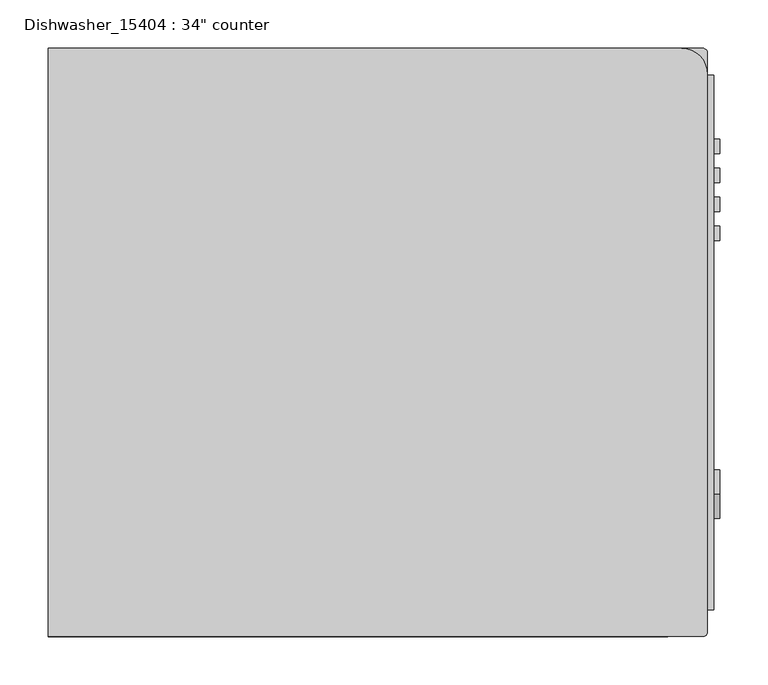
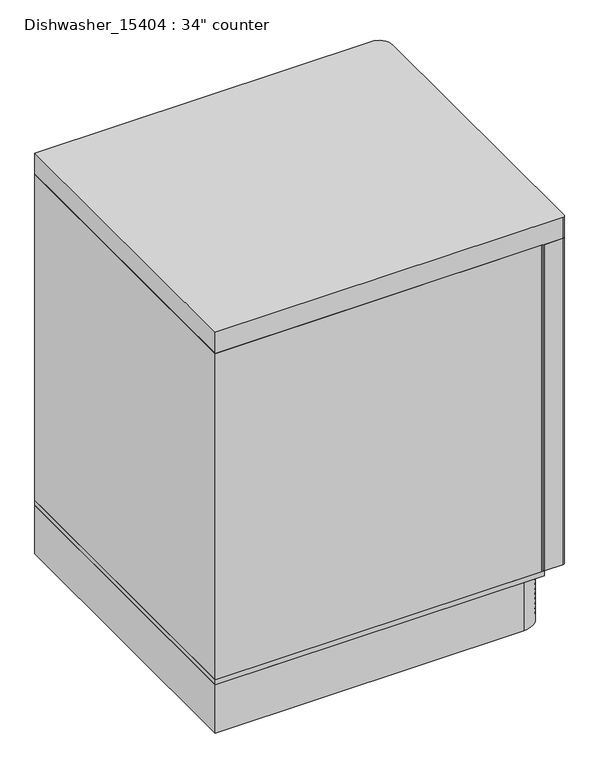
"""IFC4 building model written with IfcOpenShell, lengths in millimetres: proxy geometry."""

import ifcopenshell
import ifcopenshell.guid

model = None  # the IFC model being written
_history = None  # IfcOwnerHistory: only IFC2X3 demands one
_inside = {}  # id of a spatial element -> (the spatial element, [elements in it])
_under = {}  # id of a project, library or spatial element -> (it, [spatial elements below it])
_declared = {}  # id of a project -> (the project, [libraries it declares])
_typed = {}  # id of a type object -> (the type object, [elements of that type])
_made_of = {}  # id of a material, layer set ... -> (it, [elements and type objects made of it])


def new_model(schema):
    """Start an empty IFC model of exactly this schema.

    Asked for "IFC4X3", IfcOpenShell would pick the latest addendum, in which some entities
    have other attributes; the version numbers below select the first issue.
    IFC2X3 requires an IfcOwnerHistory on every rooted entity: one is made here for all.
    """
    global model, _history
    if schema == "IFC4X3":
        model = ifcopenshell.file(schema_version=(4, 3, 0, 0))
    else:
        model = ifcopenshell.file(schema=schema)
    _inside.clear()
    _under.clear()
    _declared.clear()
    _typed.clear()
    _made_of.clear()
    _history = None
    if model.schema == "IFC2X3":
        org = make("IfcOrganization", Name="unknown")
        user = make(
            "IfcPersonAndOrganization",
            ThePerson=make("IfcPerson", FamilyName="unknown"),
            TheOrganization=org,
        )
        app = make(
            "IfcApplication",
            ApplicationDeveloper=org,
            Version="unknown",
            ApplicationFullName="unknown",
            ApplicationIdentifier="unknown",
        )
        _history = make(
            "IfcOwnerHistory",
            OwningUser=user,
            OwningApplication=app,
            ChangeAction="ADDED",
            CreationDate=0,
        )
    return model


def make(cls, **values):
    """One entity of the class cls with the attributes given. An attribute that is None is left unset."""
    return model.create_entity(
        cls, **{name: value for name, value in values.items() if value is not None}
    )


def rooted(cls, **values):
    """An entity with a GlobalId (a new one), such as an element, a storey or a relation."""
    return make(cls, GlobalId=ifcopenshell.guid.new(), OwnerHistory=_history, **values)


def si_unit(unit_type, name, prefix=None):
    """IfcSIUnit, for example si_unit("LENGTHUNIT", "METRE", prefix="MILLI")."""
    return make("IfcSIUnit", UnitType=unit_type, Prefix=prefix, Name=name)


def assignment(units):
    """IfcUnitAssignment: the units of a project."""
    return None if units is None else make("IfcUnitAssignment", Units=units)


def point(xyz):
    """IfcCartesianPoint."""
    return None if xyz is None else make("IfcCartesianPoint", Coordinates=xyz)


def direction(xyz):
    """IfcDirection."""
    return None if xyz is None else make("IfcDirection", DirectionRatios=xyz)


def frame(location, z_axis=None, x_axis=None):
    """IfcAxis2Placement3D, a coordinate frame: its origin and axes. An axis left out is left unset."""
    return make(
        "IfcAxis2Placement3D",
        Location=point(location),
        Axis=direction(z_axis),
        RefDirection=direction(x_axis),
    )


def frame_2d(location, x_axis=None):
    """IfcAxis2Placement2D, a coordinate frame in the plane: its origin and x axis."""
    return make(
        "IfcAxis2Placement2D", Location=point(location), RefDirection=direction(x_axis)
    )


def origin():
    """The frame at (0, 0, 0) with its axes left unset."""
    return frame((0.0, 0.0, 0.0))


def place(relative_to, where):
    """IfcLocalPlacement: puts the frame where relative to a parent placement (None: the world)."""
    return make(
        "IfcLocalPlacement", PlacementRelTo=relative_to, RelativePlacement=where
    )


def context(
    kind, dimensions, precision=None, world=None, true_north=None, identifier=None
):
    """IfcGeometricRepresentationContext, for example the 3D "Model" context."""
    return make(
        "IfcGeometricRepresentationContext",
        ContextIdentifier=identifier,
        ContextType=kind,
        CoordinateSpaceDimension=dimensions,
        Precision=precision,
        WorldCoordinateSystem=world,
        TrueNorth=true_north,
    )


def project(units=None, contexts=None):
    """IfcProject with its units and contexts."""
    return rooted(
        "IfcProject",
        Name="project",
        RepresentationContexts=contexts,
        UnitsInContext=assignment(units),
    )


def spatial(cls, under=None, at=None, **own):
    """A site, building, storey or space (cls), placed at a placement, below another one or the project."""
    s = rooted(cls, ObjectPlacement=at, **own)
    if under is not None:
        _under.setdefault(under.id(), (under, []))[1].append(s)
    return s


def polyline(points):
    """IfcPolyline through the points."""
    return make("IfcPolyline", Points=[point(p) for p in points])


def circle_curve(where, radius):
    """IfcCircle in the frame where."""
    return make("IfcCircle", Position=where, Radius=radius)


def trimmed(basis, trim1, trim2, sense, master):
    """IfcTrimmedCurve: the piece of a basis curve between two trims."""
    return make(
        "IfcTrimmedCurve",
        BasisCurve=basis,
        Trim1=trim1,
        Trim2=trim2,
        SenseAgreement=sense,
        MasterRepresentation=master,
    )


def segment(curve, same_sense, transition):
    """IfcCompositeCurveSegment."""
    return make(
        "IfcCompositeCurveSegment",
        Transition=transition,
        SameSense=same_sense,
        ParentCurve=curve,
    )


def composite_curve(segments, self_intersect=None):
    """IfcCompositeCurve: segments joined end to end."""
    return make("IfcCompositeCurve", Segments=segments, SelfIntersect=self_intersect)


def outline(outer, holes=None, kind="AREA"):
    """IfcArbitraryClosedProfileDef: a profile drawn as a closed curve; with holes, ...WithVoids."""
    if holes is None:
        return make("IfcArbitraryClosedProfileDef", ProfileType=kind, OuterCurve=outer)
    return make(
        "IfcArbitraryProfileDefWithVoids",
        ProfileType=kind,
        OuterCurve=outer,
        InnerCurves=holes,
    )


def extrude(swept, where, along, depth):
    """IfcExtrudedAreaSolid: the profile swept, set in the frame where, extruded along a direction by depth."""
    return make(
        "IfcExtrudedAreaSolid",
        SweptArea=swept,
        Position=where,
        ExtrudedDirection=direction(along),
        Depth=depth,
    )


def shape(context_of_items, identifier, shape_type, items):
    """IfcShapeRepresentation: the items that make up one representation, for example the "Body"."""
    return make(
        "IfcShapeRepresentation",
        ContextOfItems=context_of_items,
        RepresentationIdentifier=identifier,
        RepresentationType=shape_type,
        Items=items,
    )


def source(mapping_origin, context_of_items, identifier, shape_type, items):
    """IfcRepresentationMap: a shape defined once, which mapped items show again and again."""
    return make(
        "IfcRepresentationMap",
        MappingOrigin=mapping_origin,
        MappedRepresentation=shape(context_of_items, identifier, shape_type, items),
    )


def transform(
    local_origin,
    x_axis=None,
    y_axis=None,
    z_axis=None,
    scale=None,
    scale2=None,
    scale3=None,
    uniform=True,
):
    """IfcCartesianTransformationOperator3D, or its non-uniform kind. x_axis, y_axis, z_axis: its Axis1, 2, 3."""
    if uniform:
        return make(
            "IfcCartesianTransformationOperator3D",
            Axis1=direction(x_axis),
            Axis2=direction(y_axis),
            LocalOrigin=point(local_origin),
            Scale=scale,
            Axis3=direction(z_axis),
        )
    return make(
        "IfcCartesianTransformationOperator3DnonUniform",
        Axis1=direction(x_axis),
        Axis2=direction(y_axis),
        LocalOrigin=point(local_origin),
        Scale=scale,
        Axis3=direction(z_axis),
        Scale2=scale2,
        Scale3=scale3,
    )


def mapped(mapping_source, mapping_target):
    """IfcMappedItem: shows the shape of a source again, moved by a transform."""
    return make(
        "IfcMappedItem", MappingSource=mapping_source, MappingTarget=mapping_target
    )


def made_of(thing, what):
    """Note that an element or type object is made of a material, layer set ...; save() writes the relation."""
    if what is not None:
        _made_of.setdefault(what.id(), (what, []))[1].append(thing)
    return thing


def element(
    cls,
    number,
    at=None,
    inside=None,
    cuts=None,
    type_object=None,
    material=None,
    context=None,
    identifier="Body",
    shape_type=None,
    held_by="IfcProductDefinitionShape",
    body=None,
    shapes=None,
    **own,
):
    """One element of the class cls, such as IfcWall. Its Tag is "e" and its number.

    at: its placement. inside: the storey or other place that contains it. cuts: it is an
    opening in that element (IfcRelVoidsElement). A single representation is given by context,
    identifier, shape_type and body (its items); several are given by shapes. held_by: the class
    of the entity that holds the representations. save() writes the other relations.
    """
    e = rooted(cls, Tag="e%d" % number, ObjectPlacement=at, **own)
    if body is not None:
        shapes = [shape(context, identifier, shape_type, body)]
    if shapes is not None:
        e.Representation = make(held_by, Representations=shapes)
    if inside is not None:
        _inside.setdefault(inside.id(), (inside, []))[1].append(e)
    if cuts is not None:
        rooted(
            "IfcRelVoidsElement", RelatingBuildingElement=cuts, RelatedOpeningElement=e
        )
    if type_object is not None:
        _typed.setdefault(type_object.id(), (type_object, []))[1].append(e)
    return made_of(e, material)


def aggregate(whole, parts):
    """IfcRelAggregates: a whole, such as a stair, and the parts it consists of."""
    return rooted("IfcRelAggregates", RelatingObject=whole, RelatedObjects=parts)


def save(model, path):
    """Write the relations noted so far, then the file.

    IfcRelAggregates (storeys below a building ...), IfcRelContainedInSpatialStructure (elements
    in a storey), IfcRelDefinesByType, IfcRelAssociatesMaterial and IfcRelDeclares: one each for
    every whole, place, type object, material and project.
    """
    for whole, parts in _under.values():
        aggregate(whole, parts)
    for where, things in _inside.values():
        rooted(
            "IfcRelContainedInSpatialStructure",
            RelatedElements=things,
            RelatingStructure=where,
        )
    for kind, things in _typed.values():
        rooted("IfcRelDefinesByType", RelatedObjects=things, RelatingType=kind)
    for what, things in _made_of.values():
        rooted("IfcRelAssociatesMaterial", RelatedObjects=things, RelatingMaterial=what)
    for by, libraries in _declared.values():
        rooted("IfcRelDeclares", RelatingContext=by, RelatedDefinitions=libraries)
    model.write(path)


def plane_surface(at):
    """IfcPlane: the flat surface through the origin of the frame at, square to its z axis."""
    return make("IfcPlane", Position=at)


def cylinder_surface(at, radius):
    """IfcCylindricalSurface: all points at the distance radius from the z axis of the frame at."""
    return make("IfcCylindricalSurface", Position=at, Radius=radius)


def advanced_brep(points, edges, surfaces, faces):
    """IfcAdvancedBrep: a solid bounded by faces that lie on surfaces and meet in shared edges.

    An edge is (start, end): straight between two places in points (the first is 0);
    or (start, end, curve); or (start, end, curve, False) where it runs against its curve.
    A face is (place in surfaces, loops), or (place, loops, False) where it looks against
    its surface's normal. A loop lists edges by number (the first is 1), with a minus sign
    where the edge is run from its end to its start. The first loop is the outer one.
    """
    corners = [point(p) for p in points]
    vertices = [make("IfcVertexPoint", VertexGeometry=c) for c in corners]
    made = []
    for start, end, *more in edges:
        made.append(
            make(
                "IfcEdgeCurve",
                EdgeStart=vertices[start],
                EdgeEnd=vertices[end],
                EdgeGeometry=more[0] if more else make("IfcPolyline", Points=[corners[start], corners[end]]),
                SameSense=more[1] if len(more) > 1 else True,
            )
        )
    hull = []
    for where, loops, *sense in faces:
        bounds = []
        for j, loop in enumerate(loops):
            ring = [make("IfcOrientedEdge", EdgeElement=made[abs(k) - 1], Orientation=k > 0) for k in loop]
            bounds.append(
                make(
                    "IfcFaceOuterBound" if j == 0 else "IfcFaceBound",
                    Bound=make("IfcEdgeLoop", EdgeList=ring),
                    Orientation=True,
                )
            )
        hull.append(make("IfcAdvancedFace", Bounds=bounds, FaceSurface=surfaces[where], SameSense=sense[0] if sense else True))
    return make("IfcAdvancedBrep", Outer=make("IfcClosedShell", CfsFaces=hull))


def proxy_e1c3c540(model_context):
    return source(origin(), model_context, "Body", "SolidModel", [
        extrude(outline(composite_curve([segment(trimmed(circle_curve(frame_2d((147.53066, 741.5840355)), 25.0), [point((147.53066, 716.5840355))], [point((147.53066, 766.5840355))], False, "CARTESIAN"), True, "CONTINUOUS"), segment(trimmed(circle_curve(frame_2d((147.53066, 741.5840355)), 25.0), [point((147.53066, 766.5840355))], [point((147.53066, 716.5840355))], False, "CARTESIAN"), True, "CONTINUOUS")], self_intersect=False)), frame((688.975, 0.0, 0.0), z_axis=(1.0, 0.0, 0.0), x_axis=(0.0, 1.0, 0.0)), (0.0, 0.0, 1.0), 6.35),
        extrude(outline(polyline([(688.975, 410.2108979), (688.975, 425.2108979), (695.325, 425.2108979), (695.325, 410.2108979), (688.975, 410.2108979)])), frame((0.0, 0.0, 745.4030607), z_axis=(0.0, 0.0, 1.0), x_axis=(1.0, 0.0, 0.0)), (0.0, 0.0, 1.0), 15.0),
        extrude(outline(polyline([(688.975, 440.2108979), (688.975, 455.2108979), (695.325, 455.2108979), (695.325, 440.2108979), (688.975, 440.2108979)])), frame((0.0, 0.0, 745.4030607), z_axis=(0.0, 0.0, 1.0), x_axis=(1.0, 0.0, 0.0)), (0.0, 0.0, 1.0), 15.0),
        extrude(outline(polyline([(688.975, 470.2108979), (688.975, 485.2108979), (695.325, 485.2108979), (695.325, 470.2108979), (688.975, 470.2108979)])), frame((0.0, 0.0, 745.4030607), z_axis=(0.0, 0.0, 1.0), x_axis=(1.0, 0.0, 0.0)), (0.0, 0.0, 1.0), 15.0),
        extrude(outline(polyline([(688.975, 500.2108979), (688.975, 515.2108979), (695.325, 515.2108979), (695.325, 500.2108979), (688.975, 500.2108979)])), frame((0.0, 0.0, 745.4030607), z_axis=(0.0, 0.0, 1.0), x_axis=(1.0, 0.0, 0.0)), (0.0, 0.0, 1.0), 15.0),
        extrude(outline(composite_curve([segment(polyline([(512.7209143, 694.5980964), (96.8794309, 694.5980964)]), True, "CONTINUOUS"), segment(trimmed(circle_curve(frame_2d((96.8794309, 729.5980964)), 35.0), [point((96.8794309, 694.5980964))], [point((66.2677412, 712.6297597))], False, "CARTESIAN"), True, "CONTINUOUS"), segment(polyline([(66.2677412, 712.6297597), (27.7608134, 782.0980964), (581.8395319, 782.0980964), (543.3326041, 712.6297597)]), True, "CONTINUOUS"), segment(trimmed(circle_curve(frame_2d((512.7209143, 729.5980964)), 35.0), [point((543.3326041, 712.6297597))], [point((512.7209143, 694.5980964))], False, "CARTESIAN"), True, "CONTINUOUS")], self_intersect=False)), frame((638.175, 0.0, 0.0), z_axis=(1.0, 0.0, 0.0), x_axis=(0.0, 1.0, 0.0)), (0.0, 0.0, 1.0), 50.8),
        extrude(outline(composite_curve([segment(polyline([(0.0, 609.6), (636.35, 609.6)]), True, "CONTINUOUS"), segment(trimmed(circle_curve(frame_2d((636.35, 604.6)), 5.0), [point((636.35, 609.6))], [point((641.35, 604.6))], False, "CARTESIAN"), True, "CONTINUOUS"), segment(polyline([(641.35, 604.6), (641.35, 5.0003453)]), True, "CONTINUOUS"), segment(trimmed(circle_curve(frame_2d((636.35, 5.0003453)), 5.0), [point((641.35, 5.0003453))], [point((636.35, 0.0003453))], False, "CARTESIAN"), True, "CONTINUOUS"), segment(polyline([(636.35, 0.0003453), (0.0, 0.0003453), (0.0, 609.6)]), True, "CONTINUOUS")], self_intersect=False)), frame((0.0, 0.0, 110.0), z_axis=(0.0, 0.0, 1.0), x_axis=(1.0, 0.0, 0.0)), (0.0, 0.0, 1.0), 672.0980964),
        extrude(outline(composite_curve([segment(polyline([(0.0, 609.6), (655.4, 609.6)]), True, "CONTINUOUS"), segment(trimmed(circle_curve(frame_2d((655.4, 582.375)), 27.225), [point((655.4, 609.6))], [point((682.625, 582.375))], False, "CARTESIAN"), True, "CONTINUOUS"), segment(polyline([(682.625, 582.375), (682.625, 5.0)]), True, "CONTINUOUS"), segment(trimmed(circle_curve(frame_2d((677.625, 5.0)), 5.0), [point((682.625, 5.0))], [point((677.625, 0.0))], False, "CARTESIAN"), True, "CONTINUOUS"), segment(polyline([(677.625, 0.0), (0.0, 0.0), (0.0, 609.6)]), True, "CONTINUOUS")], self_intersect=False)), frame((0.0, 0.0, 782.0980964), z_axis=(0.0, 0.0, 1.0), x_axis=(1.0, 0.0, 0.0)), (0.0, 0.0, 1.0), 43.4019036),
        extrude(outline(composite_curve([segment(polyline([(641.35, 609.6), (677.625, 609.6)]), True, "CONTINUOUS"), segment(trimmed(circle_curve(frame_2d((677.625, 604.6)), 5.0), [point((677.625, 609.6))], [point((682.625, 604.6))], False, "CARTESIAN"), True, "CONTINUOUS"), segment(polyline([(682.625, 604.6), (682.625, 5.0)]), True, "CONTINUOUS"), segment(trimmed(circle_curve(frame_2d((677.625, 5.0)), 5.0), [point((682.625, 5.0))], [point((677.625, 0.0))], False, "CARTESIAN"), True, "CONTINUOUS"), segment(polyline([(677.625, 0.0), (641.35, 0.0), (641.35, 609.6)]), True, "CONTINUOUS")], self_intersect=False)), frame((0.0, 0.0, 110.0), z_axis=(0.0, 0.0, 1.0), x_axis=(1.0, 0.0, 0.0)), (0.0, 0.0, 1.0), 672.0980964),
        extrude(outline(polyline([(0.0, 609.6), (641.35, 609.6), (641.35, 0.0), (0.0, 0.0), (0.0, 609.6)])), frame((0.0, 0.0, 100.0), z_axis=(0.0, 0.0, 1.0), x_axis=(1.0, 0.0, 0.0)), (0.0, 0.0, 1.0), 10.0),
        advanced_brep(
        [(0.0, 609.6, 100.0), (0.0, 0.0, 100.0), (601.35, 0.0, 100.0), (641.35, 40.0, 100.0), (641.35, 569.6, 100.0), (601.35, 609.6, 100.0), (0.0, 609.6, 0.0), (601.35, 609.6, 0.0), (641.35, 569.6, 0.0), (641.35, 40.0, 0.0), (601.35, 0.0, 0.0), (0.0, 0.0, 0.0), (641.35, 40.0, 16.3757772), (628.65, 10.7645763, 16.3757772), (628.65, 10.7645763, 21.3757772), (641.35, 40.0, 21.3757772), (641.35, 40.0, 26.2238547), (628.65, 10.7645763, 26.2238547), (628.65, 10.7645763, 31.2238547), (641.35, 40.0, 31.2238547), (641.35, 40.0, 36.2238547), (628.65, 10.7645763, 36.2238547), (628.65, 10.7645763, 41.2238547), (641.35, 40.0, 41.2238547), (641.35, 40.0, 46.2238547), (628.65, 10.7645763, 46.2238547), (628.65, 10.7645763, 51.2238547), (641.35, 40.0, 51.2238547), (641.35, 40.0, 56.2238547), (628.65, 10.7645763, 56.2238547), (628.65, 10.7645763, 61.2238547), (641.35, 40.0, 61.2238547), (641.35, 40.0, 66.2238547), (628.65, 10.7645763, 66.2238547), (628.65, 10.7645763, 71.2238547), (641.35, 40.0, 71.2238547), (641.35, 40.0, 76.2238547), (628.65, 10.7645763, 76.2238547), (628.65, 10.7645763, 81.2238547), (641.35, 40.0, 81.2238547), (641.35, 40.0, 86.2238547), (628.65, 10.7645763, 86.2238547), (628.65, 10.7645763, 91.2238547), (641.35, 40.0, 91.2238547), (641.35, 569.6, 91.2238547), (641.35, 569.6, 16.3757772), (641.35, 569.6, 21.3757772), (641.35, 569.6, 26.2238547), (641.35, 569.6, 31.2238547), (641.35, 569.6, 36.2238547), (641.35, 569.6, 41.2238547), (641.35, 569.6, 46.2238547), (641.35, 569.6, 51.2238547), (641.35, 569.6, 56.2238547), (641.35, 569.6, 61.2238547), (641.35, 569.6, 66.2238547), (641.35, 569.6, 71.2238547), (641.35, 569.6, 76.2238547), (641.35, 569.6, 81.2238547), (641.35, 569.6, 86.2238547), (628.65, 598.8354237, 91.2238547), (628.65, 598.8354237, 86.2238547), (628.65, 598.8354237, 81.2238547), (628.65, 598.8354237, 76.2238547), (628.65, 598.8354237, 71.2238547), (628.65, 598.8354237, 66.2238547), (628.65, 598.8354237, 61.2238547), (628.65, 598.8354237, 56.2238547), (628.65, 598.8354237, 51.2238547), (628.65, 598.8354237, 46.2238547), (628.65, 598.8354237, 41.2238547), (628.65, 598.8354237, 36.2238547), (628.65, 598.8354237, 31.2238547), (628.65, 598.8354237, 26.2238547), (628.65, 598.8354237, 21.3757772), (628.65, 598.8354237, 16.3757772)],
        [
            (0, 1),
            (1, 2),
            (2, 3, circle_curve(frame((601.35, 40.0, 100.0), z_axis=(0.0, 0.0, 1.0), x_axis=(1.0, 0.0, 0.0)), 40.0)),
            (3, 4),
            (4, 5, circle_curve(frame((601.35, 569.6, 100.0), z_axis=(0.0, 0.0, 1.0), x_axis=(1.0, 0.0, 0.0)), 40.0)),
            (5, 0),
            (6, 7),
            (7, 8, circle_curve(frame((601.35, 569.6, 0.0), z_axis=(0.0, 0.0, -1.0), x_axis=(1.0, 0.0, 0.0)), 40.0)),
            (8, 9),
            (9, 10, circle_curve(frame((601.35, 40.0, 0.0), z_axis=(0.0, 0.0, -1.0), x_axis=(1.0, 0.0, 0.0)), 40.0)),
            (10, 11),
            (11, 6),
            (0, 6),
            (11, 1),
            (10, 2),
            (9, 12),
            (12, 13, circle_curve(frame((601.35, 40.0, 16.3757772), z_axis=(0.0, 0.0, -1.0), x_axis=(1.0, 0.0, 0.0)), 40.0)),
            (13, 14),
            (14, 15, circle_curve(frame((601.35, 40.0, 21.3757772), z_axis=(0.0, 0.0, 1.0), x_axis=(1.0, 0.0, 0.0)), 40.0)),
            (15, 16),
            (16, 17, circle_curve(frame((601.35, 40.0, 26.2238547), z_axis=(0.0, 0.0, -1.0), x_axis=(1.0, 0.0, 0.0)), 40.0)),
            (17, 18),
            (18, 19, circle_curve(frame((601.35, 40.0, 31.2238547), z_axis=(0.0, 0.0, 1.0), x_axis=(1.0, 0.0, 0.0)), 40.0)),
            (19, 20),
            (20, 21, circle_curve(frame((601.35, 40.0, 36.2238547), z_axis=(0.0, 0.0, -1.0), x_axis=(1.0, 0.0, 0.0)), 40.0)),
            (21, 22),
            (22, 23, circle_curve(frame((601.35, 40.0, 41.2238547), z_axis=(0.0, 0.0, 1.0), x_axis=(1.0, 0.0, 0.0)), 40.0)),
            (23, 24),
            (24, 25, circle_curve(frame((601.35, 40.0, 46.2238547), z_axis=(0.0, 0.0, -1.0), x_axis=(1.0, 0.0, 0.0)), 40.0)),
            (25, 26),
            (26, 27, circle_curve(frame((601.35, 40.0, 51.2238547), z_axis=(0.0, 0.0, 1.0), x_axis=(1.0, 0.0, 0.0)), 40.0)),
            (27, 28),
            (28, 29, circle_curve(frame((601.35, 40.0, 56.2238547), z_axis=(0.0, 0.0, -1.0), x_axis=(1.0, 0.0, 0.0)), 40.0)),
            (29, 30),
            (30, 31, circle_curve(frame((601.35, 40.0, 61.2238547), z_axis=(0.0, 0.0, 1.0), x_axis=(1.0, 0.0, 0.0)), 40.0)),
            (31, 32),
            (32, 33, circle_curve(frame((601.35, 40.0, 66.2238547), z_axis=(0.0, 0.0, -1.0), x_axis=(1.0, 0.0, 0.0)), 40.0)),
            (33, 34),
            (34, 35, circle_curve(frame((601.35, 40.0, 71.2238547), z_axis=(0.0, 0.0, 1.0), x_axis=(1.0, 0.0, 0.0)), 40.0)),
            (35, 36),
            (36, 37, circle_curve(frame((601.35, 40.0, 76.2238547), z_axis=(0.0, 0.0, -1.0), x_axis=(1.0, 0.0, 0.0)), 40.0)),
            (37, 38),
            (38, 39, circle_curve(frame((601.35, 40.0, 81.2238547), z_axis=(0.0, 0.0, 1.0), x_axis=(1.0, 0.0, 0.0)), 40.0)),
            (39, 40),
            (40, 41, circle_curve(frame((601.35, 40.0, 86.2238547), z_axis=(0.0, 0.0, -1.0), x_axis=(1.0, 0.0, 0.0)), 40.0)),
            (41, 42),
            (42, 43, circle_curve(frame((601.35, 40.0, 91.2238547), z_axis=(0.0, 0.0, 1.0), x_axis=(1.0, 0.0, 0.0)), 40.0)),
            (43, 3),
            (43, 44),
            (44, 4),
            (8, 45),
            (45, 12),
            (15, 46),
            (46, 47),
            (47, 16),
            (19, 48),
            (48, 49),
            (49, 20),
            (23, 50),
            (50, 51),
            (51, 24),
            (27, 52),
            (52, 53),
            (53, 28),
            (31, 54),
            (54, 55),
            (55, 32),
            (35, 56),
            (56, 57),
            (57, 36),
            (39, 58),
            (58, 59),
            (59, 40),
            (44, 60, circle_curve(frame((601.35, 569.6, 91.2238547), z_axis=(0.0, 0.0, 1.0), x_axis=(1.0, 0.0, 0.0)), 40.0)),
            (60, 61),
            (61, 59, circle_curve(frame((601.35, 569.6, 86.2238547), z_axis=(0.0, 0.0, -1.0), x_axis=(1.0, 0.0, 0.0)), 40.0)),
            (58, 62, circle_curve(frame((601.35, 569.6, 81.2238547), z_axis=(0.0, 0.0, 1.0), x_axis=(1.0, 0.0, 0.0)), 40.0)),
            (62, 63),
            (63, 57, circle_curve(frame((601.35, 569.6, 76.2238547), z_axis=(0.0, 0.0, -1.0), x_axis=(1.0, 0.0, 0.0)), 40.0)),
            (56, 64, circle_curve(frame((601.35, 569.6, 71.2238547), z_axis=(0.0, 0.0, 1.0), x_axis=(1.0, 0.0, 0.0)), 40.0)),
            (64, 65),
            (65, 55, circle_curve(frame((601.35, 569.6, 66.2238547), z_axis=(0.0, 0.0, -1.0), x_axis=(1.0, 0.0, 0.0)), 40.0)),
            (54, 66, circle_curve(frame((601.35, 569.6, 61.2238547), z_axis=(0.0, 0.0, 1.0), x_axis=(1.0, 0.0, 0.0)), 40.0)),
            (66, 67),
            (67, 53, circle_curve(frame((601.35, 569.6, 56.2238547), z_axis=(0.0, 0.0, -1.0), x_axis=(1.0, 0.0, 0.0)), 40.0)),
            (52, 68, circle_curve(frame((601.35, 569.6, 51.2238547), z_axis=(0.0, 0.0, 1.0), x_axis=(1.0, 0.0, 0.0)), 40.0)),
            (68, 69),
            (69, 51, circle_curve(frame((601.35, 569.6, 46.2238547), z_axis=(0.0, 0.0, -1.0), x_axis=(1.0, 0.0, 0.0)), 40.0)),
            (50, 70, circle_curve(frame((601.35, 569.6, 41.2238547), z_axis=(0.0, 0.0, 1.0), x_axis=(1.0, 0.0, 0.0)), 40.0)),
            (70, 71),
            (71, 49, circle_curve(frame((601.35, 569.6, 36.2238547), z_axis=(0.0, 0.0, -1.0), x_axis=(1.0, 0.0, 0.0)), 40.0)),
            (48, 72, circle_curve(frame((601.35, 569.6, 31.2238547), z_axis=(0.0, 0.0, 1.0), x_axis=(1.0, 0.0, 0.0)), 40.0)),
            (72, 73),
            (73, 47, circle_curve(frame((601.35, 569.6, 26.2238547), z_axis=(0.0, 0.0, -1.0), x_axis=(1.0, 0.0, 0.0)), 40.0)),
            (46, 74, circle_curve(frame((601.35, 569.6, 21.3757772), z_axis=(0.0, 0.0, 1.0), x_axis=(1.0, 0.0, 0.0)), 40.0)),
            (74, 75),
            (75, 45, circle_curve(frame((601.35, 569.6, 16.3757772), z_axis=(0.0, 0.0, -1.0), x_axis=(1.0, 0.0, 0.0)), 40.0)),
            (7, 5),
            (60, 42),
            (41, 61),
            (62, 38),
            (37, 63),
            (64, 34),
            (33, 65),
            (66, 30),
            (29, 67),
            (68, 26),
            (25, 69),
            (70, 22),
            (21, 71),
            (72, 18),
            (17, 73),
            (74, 14),
            (13, 75),
        ],
        [
            plane_surface(frame((0.0, 0.0, 100.0), z_axis=(0.0, 0.0, 1.0), x_axis=(0.0, -1.0, 0.0))),
            plane_surface(frame((0.0, 0.0, 0.0), z_axis=(0.0, 0.0, -1.0), x_axis=(0.0, 1.0, 0.0))),
            plane_surface(frame((0.0, 609.6, 100.0), z_axis=(-1.0, 0.0, 0.0), x_axis=(0.0, 0.0, -1.0))),
            plane_surface(frame((0.0, 0.0, 100.0), z_axis=(0.0, -1.0, 0.0), x_axis=(0.0, 0.0, -1.0))),
            cylinder_surface(frame((601.35, 40.0, 0.0), z_axis=(0.0, 0.0, 1.0), x_axis=(1.0, 0.0, 0.0)), 40.0),
            plane_surface(frame((641.35, 40.0, 100.0), z_axis=(1.0, 0.0, 0.0), x_axis=(0.0, 0.0, -1.0))),
            cylinder_surface(frame((601.35, 569.6, 0.0), z_axis=(0.0, 0.0, 1.0), x_axis=(1.0, 0.0, 0.0)), 40.0),
            plane_surface(frame((601.35, 609.6, 100.0), z_axis=(0.0, 1.0, 0.0), x_axis=(0.0, 0.0, -1.0))),
            plane_surface(frame((628.65, 0.0, 91.2238547), z_axis=(1.0, 0.0, 0.0), x_axis=(0.0, 1.0, 0.0))),
            plane_surface(frame((666.75, 609.6, 91.2238547), z_axis=(0.0, 0.0, -1.0), x_axis=(-1.0, 0.0, 0.0))),
            plane_surface(frame((666.75, 0.0, 86.2238547), z_axis=(0.0, 0.0, 1.0), x_axis=(-1.0, 0.0, 0.0))),
            plane_surface(frame((666.75, 609.6, 81.2238547), z_axis=(0.0, 0.0, -1.0), x_axis=(-1.0, 0.0, 0.0))),
            plane_surface(frame((666.75, 0.0, 76.2238547), z_axis=(0.0, 0.0, 1.0), x_axis=(-1.0, 0.0, 0.0))),
            plane_surface(frame((666.75, 609.6, 71.2238547), z_axis=(0.0, 0.0, -1.0), x_axis=(-1.0, 0.0, 0.0))),
            plane_surface(frame((666.75, 0.0, 66.2238547), z_axis=(0.0, 0.0, 1.0), x_axis=(-1.0, 0.0, 0.0))),
            plane_surface(frame((666.75, 609.6, 61.2238547), z_axis=(0.0, 0.0, -1.0), x_axis=(-1.0, 0.0, 0.0))),
            plane_surface(frame((666.75, 0.0, 56.2238547), z_axis=(0.0, 0.0, 1.0), x_axis=(-1.0, 0.0, 0.0))),
            plane_surface(frame((666.75, 609.6, 51.2238547), z_axis=(0.0, 0.0, -1.0), x_axis=(-1.0, 0.0, 0.0))),
            plane_surface(frame((666.75, 0.0, 46.2238547), z_axis=(0.0, 0.0, 1.0), x_axis=(-1.0, 0.0, 0.0))),
            plane_surface(frame((666.75, 609.6, 41.2238547), z_axis=(0.0, 0.0, -1.0), x_axis=(-1.0, 0.0, 0.0))),
            plane_surface(frame((666.75, 0.0, 36.2238547), z_axis=(0.0, 0.0, 1.0), x_axis=(-1.0, 0.0, 0.0))),
            plane_surface(frame((666.75, 609.6, 31.2238547), z_axis=(0.0, 0.0, -1.0), x_axis=(-1.0, 0.0, 0.0))),
            plane_surface(frame((666.75, 0.0, 26.2238547), z_axis=(0.0, 0.0, 1.0), x_axis=(-1.0, 0.0, 0.0))),
            plane_surface(frame((666.75, 609.6, 21.3757772), z_axis=(0.0, 0.0, -1.0), x_axis=(-1.0, 0.0, 0.0))),
            plane_surface(frame((666.75, 0.0, 16.3757772), z_axis=(0.0, 0.0, 1.0), x_axis=(-1.0, 0.0, 0.0))),
        ],
        [
            (0, [[1, 2, 3, 4, 5, 6]]),
            (1, [[7, 8, 9, 10, 11, 12]]),
            (2, [[-1, 13, -12, 14]]),
            (3, [[-2, -14, -11, 15]]),
            (4, [[-3, -15, -10, 16, 17, 18, 19, 20, 21, 22, 23, 24, 25, 26, 27, 28, 29, 30, 31, 32, 33, 34, 35, 36, 37, 38, 39, 40, 41, 42, 43, 44, 45, 46, 47, 48]]),
            (5, [[-4, -48, 49, 50]]),
            (5, [[-9, 51, 52, -16]]),
            (5, [[-20, 53, 54, 55]]),
            (5, [[-24, 56, 57, 58]]),
            (5, [[-28, 59, 60, 61]]),
            (5, [[-32, 62, 63, 64]]),
            (5, [[-36, 65, 66, 67]]),
            (5, [[-40, 68, 69, 70]]),
            (5, [[-44, 71, 72, 73]]),
            (6, [[-5, -50, 74, 75, 76, -72, 77, 78, 79, -69, 80, 81, 82, -66, 83, 84, 85, -63, 86, 87, 88, -60, 89, 90, 91, -57, 92, 93, 94, -54, 95, 96, 97, -51, -8, 98]]),
            (7, [[-6, -98, -7, -13]]),
            (8, [[99, -46, 100, -75]]),
            (8, [[101, -42, 102, -78]]),
            (8, [[103, -38, 104, -81]]),
            (8, [[105, -34, 106, -84]]),
            (8, [[107, -30, 108, -87]]),
            (8, [[109, -26, 110, -90]]),
            (8, [[111, -22, 112, -93]]),
            (8, [[113, -18, 114, -96]]),
            (9, [[-99, -74, -49, -47]]),
            (10, [[-100, -45, -73, -76]]),
            (11, [[-101, -77, -71, -43]]),
            (12, [[-102, -41, -70, -79]]),
            (13, [[-103, -80, -68, -39]]),
            (14, [[-104, -37, -67, -82]]),
            (15, [[-105, -83, -65, -35]]),
            (16, [[-106, -33, -64, -85]]),
            (17, [[-107, -86, -62, -31]]),
            (18, [[-108, -29, -61, -88]]),
            (19, [[-109, -89, -59, -27]]),
            (20, [[-110, -25, -58, -91]]),
            (21, [[-111, -92, -56, -23]]),
            (22, [[-112, -21, -55, -94]]),
            (23, [[-113, -95, -53, -19]]),
            (24, [[-114, -17, -52, -97]]),
        ],
    ),
    ])


if __name__ == "__main__":
    model = new_model("IFC4")
    model_context = context("Model", 3, world=origin())
    ifc_project = project(units=[si_unit("LENGTHUNIT", "METRE", prefix="MILLI")], contexts=[model_context])
    site = spatial("IfcSite", under=ifc_project)
    building = spatial("IfcBuilding", under=site)
    placement = place(None, origin())
    proxy_shape = proxy_e1c3c540(model_context)
    element("IfcBuildingElementProxy", 1, Name="Dishwasher_15404 : 34\" counter", ObjectType="Dishwasher_15404 : 34\" counter", at=placement, inside=building, context=model_context, shape_type="MappedRepresentation", body=[
        mapped(proxy_shape, transform((0.0, 0.0, 0.0), x_axis=(1.0, 0.0, 0.0), y_axis=(0.0, 1.0, 0.0), z_axis=(0.0, 0.0, 1.0))),
    ])
    save(model, "model.ifc")

# Revit data of these elements
# Type "Dishwasher_15404 : 34\" counter"
#   Width = 2' - 0"
#   Height = 2' - 8 1/2"
#   Depth = 2' - 0"
